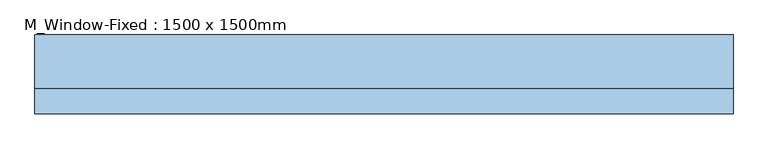
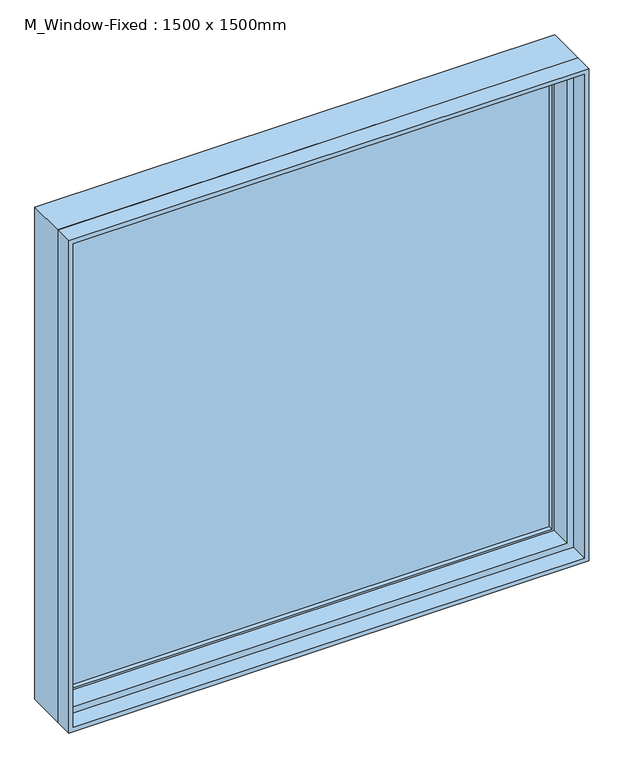
"""IFC4 building model written with IfcOpenShell, lengths in millimetres: window geometry, M_Window-Fixed : 1500 x 1500mm."""

from ifc_helpers import new_model, si_unit, frame, origin, place, context, project, spatial, polyline, outline, extrude, faceted_brep, source, transform, mapped, element, save


def m_window_fixed_1500_x_1500mm_80caa23a(model_context):
    return source(origin(), model_context, "Body", "SolidModel", [
        faceted_brep([(750.0, -20.25, 2400.0), (750.0, 94.05, 2400.0), (-750.0, 94.05, 2400.0), (-750.0, -20.25, 2400.0), (-750.0, 94.05, 900.0), (-750.0, -20.25, 900.0), (750.0, 94.05, 900.0), (750.0, -20.25, 900.0), (718.25, -20.25, 2368.25), (718.25, -20.25, 931.75), (-718.25, -20.25, 931.75), (-718.25, -20.25, 2368.25), (-737.3, 94.05, 2387.3), (-737.3, 94.05, 912.7), (737.3, 94.05, 912.7), (737.3, 94.05, 2387.3), (718.25, 43.25, 2368.25), (-718.25, 43.25, 2368.25), (737.3, 43.25, 2387.3), (-737.3, 43.25, 2387.3), (-718.25, 43.25, 931.75), (-737.3, 43.25, 912.7), (718.25, 43.25, 931.75), (737.3, 43.25, 912.7)], [[[0, 1, 2, 3]], [[3, 2, 4, 5]], [[5, 4, 6, 7]], [[3, 5, 7, 0], [8, 9, 10, 11]], [[7, 6, 1, 0]], [[1, 6, 4, 2], [12, 13, 14, 15]], [[16, 8, 11, 17]], [[15, 18, 19, 12]], [[17, 11, 10, 20]], [[12, 19, 21, 13]], [[20, 10, 9, 22]], [[13, 21, 23, 14]], [[22, 9, 8, 16]], [[18, 23, 21, 19], [17, 20, 22, 16]], [[14, 23, 18, 15]]]),
        extrude(outline(polyline([(2400.0, -750.0), (900.0, -750.0), (900.0, 750.0), (2400.0, 750.0), (2400.0, -750.0)]), holes=[polyline([(2387.3, 737.3), (912.7, 737.3), (912.7, -737.3), (2387.3, -737.3), (2387.3, 737.3)])]), frame((0.0, -75.0, 0.0), z_axis=(0.0, 1.0, 0.0), x_axis=(0.0, 0.0, 1.0)), (0.0, 0.0, 1.0), 54.75),
        extrude(outline(polyline([(912.7, 737.3), (2387.3, 737.3), (2387.3, -737.3), (912.7, -737.3), (912.7, 737.3)]), holes=[polyline([(938.1, -711.9), (2361.9, -711.9), (2361.9, 711.9), (938.1, 711.9), (938.1, -711.9)])]), frame((0.0, 43.25, 0.0), z_axis=(0.0, 1.0, 0.0), x_axis=(0.0, 0.0, 1.0)), (0.0, 0.0, 1.0), 44.45),
        extrude(outline(polyline([(711.9, 75.0), (711.9, 68.65), (-711.9, 68.65), (-711.9, 75.0), (711.9, 75.0)])), frame((0.0, 0.0, 938.1), z_axis=(0.0, 0.0, 1.0), x_axis=(1.0, 0.0, 0.0)), (0.0, 0.0, 1.0), 1423.8),
        extrude(outline(polyline([(-711.9, 55.95), (-711.9, 62.3), (711.9, 62.3), (711.9, 55.95), (-711.9, 55.95)])), frame((0.0, 0.0, 938.1), z_axis=(0.0, 0.0, 1.0), x_axis=(1.0, 0.0, 0.0)), (0.0, 0.0, 1.0), 1423.8),
    ])


if __name__ == "__main__":
    model = new_model("IFC4")
    model_context = context("Model", 3, world=origin())
    ifc_project = project(units=[si_unit("LENGTHUNIT", "METRE", prefix="MILLI")], contexts=[model_context])
    site = spatial("IfcSite", under=ifc_project)
    building = spatial("IfcBuilding", under=site)
    placement = place(None, origin())
    m_window_fixed_1500_x_1500mm_shape = m_window_fixed_1500_x_1500mm_80caa23a(model_context)
    element("IfcWindow", 1, ObjectType="M_Window-Fixed : 1500 x 1500mm", at=placement, inside=building, context=model_context, shape_type="MappedRepresentation", body=[
        mapped(m_window_fixed_1500_x_1500mm_shape, transform((0.0, 0.0, 0.0), x_axis=(1.0, 0.0, 0.0), y_axis=(0.0, 1.0, 0.0), z_axis=(0.0, 0.0, 1.0))),
    ])
    save(model, "model.ifc")

# Revit data of these elements
# Type "M_Window-Fixed : 1500 x 1500mm"
#   Type Mark = "39"
#   Fire Rating = "0.5h"
#   Assembly Code = "B2020100"
#   Analytic Construction = "Double glazing - domestic"
#   Window Inset [instance default] = 0 mm
#   Wall Thickness [instance default] = 150 mm
#   Visual Light Transmittance = 0.81
#   Thermal Resistance (R) = 0.319569 (m²·K)/W
#   Solar Heat Gain Coefficient = 0.76
#   Rough Width = 1515 mm
#   Rough Height = 1515 mm
#   Interior Wall Closure [instance default] = 54.75 mm
#   Height = 1500 mm
#   Heat Transfer Coefficient (U) = 3.12929 W/(m²·K)
#   Frame Extension [instance default] = 6.35 mm
#   Exterior Wall Closure [instance default] = 31.75 mm
#   Extension Jamb [instance default] = 54.75 mm
#   Default Sill Height = 900 mm
#   Width = 1500 mm
#   Muntin Visibility = yes
#   Interior Trim Visibility [instance default] = yes
#   Exterior Trim Visibility [instance default] = yes
#   Extension Jamb Visibility [instance default] = yes
#   Muntin Pattern = M_Muntin Pattern_2x2 : M_Muntin Pattern_2x2
#   Interior Trim Material = Wood - Stained
#   Interior Trim = M_Trim-Window-Interior-Flat : Picture Frame
#   Interior Frame Material = Wood - Stained
#   Glass Panel Material = Glass
#   Exterior Trim Material = Clad - White
#   Exterior Trim = M_Trim-Window-Exterior-Flat : with Sill
#   Exterior Frame Material = Clad - White
#   Wall Closure = (empty or 0)
# Element 1 (IfcWindow, "M_Window-Fixed : 1500 x 1500mm")
#   Materials on its faces: "Wood - Stained", "Glass", "Clad - White"
# Materials
#   "Wood - Stained": class "Wood", colour RGB 173 132 96, transparency 0, Cost = 0
#   "Glass": class "Glass", colour RGB 245 245 243, transparency 1, Description = "Soda Lime Glass", Cost = 0
#   "Clad - White": class "Wood", colour RGB 245 245 243, transparency 0, Cost = 0
